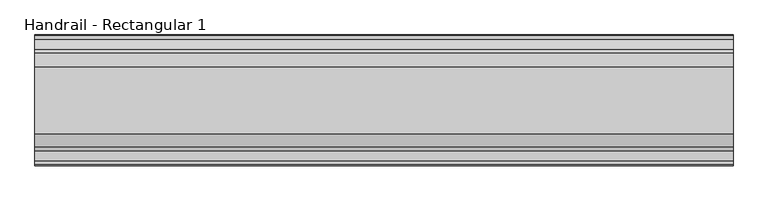
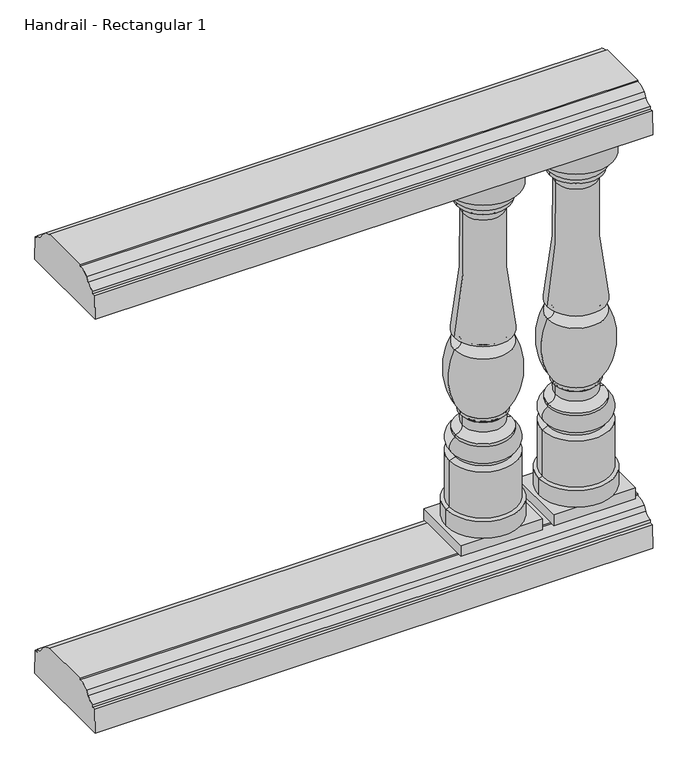
"""IFC4 building model written with IfcOpenShell, lengths in millimetres: railing geometry, Handrail - Rectangular 1."""

from ifc_helpers import new_model, si_unit, point, frame, frame_2d, origin, place, context, project, spatial, polyline, circle_curve, ellipse_curve, trimmed, segment, composite_curve, outline, extrude, source, transform, mapped, element, save
from ifc_brep_helpers import plane_surface, cylinder_surface, revolved_surface, advanced_brep


def handrail_rectangular_1_0a93f58a(model_context):
    return source(origin(), model_context, "Body", "SolidModel", [
        extrude(outline(composite_curve([segment(trimmed(circle_curve(frame_2d((-1771.1852268, 1045.36875)), 19.84375), [point((-1771.1852268, 1025.525))], [point((-1754.064785, 1035.3355607))], True, "CARTESIAN"), True, "CONTINUOUS"), segment(polyline([(-1754.064785, 1035.3355607), (-1747.604713, 1044.7951059)]), True, "CONTINUOUS"), segment(trimmed(circle_curve(frame_2d((-1723.5602268, 1018.38125)), 35.71875), [point((-1747.604713, 1044.7951059))], [point((-1723.5602268, 1054.1))], False, "CARTESIAN"), True, "CONTINUOUS"), segment(polyline([(-1723.5602268, 1054.1), (-1723.5602268, 1057.275), (-1607.6727268, 1057.275), (-1607.6727268, 1054.1)]), True, "CONTINUOUS"), segment(trimmed(circle_curve(frame_2d((-1607.6727268, 1018.38125)), 35.71875), [point((-1607.6727268, 1054.1))], [point((-1583.6282406, 1044.7951059))], False, "CARTESIAN"), True, "CONTINUOUS"), segment(polyline([(-1583.6282406, 1044.7951059), (-1577.1681686, 1035.3355607)]), True, "CONTINUOUS"), segment(trimmed(circle_curve(frame_2d((-1560.0477268, 1045.36875)), 19.84375), [point((-1577.1681686, 1035.3355607))], [point((-1560.0477268, 1025.525))], True, "CARTESIAN"), True, "CONTINUOUS"), segment(polyline([(-1560.0477268, 1025.525), (-1560.0477268, 1019.175), (-1552.9039768, 1019.175), (-1551.3164768, 965.2), (-1779.9164768, 965.2), (-1778.3289768, 1019.175), (-1771.1852268, 1019.175), (-1771.1852268, 1025.525)]), True, "CONTINUOUS")], self_intersect=False)), frame((6512.4521895, 0.0, 0.0), z_axis=(1.0, 0.0, 0.0), x_axis=(0.0, 1.0, 0.0)), (0.0, 0.0, 1.0), 1219.2),
        extrude(outline(composite_curve([segment(trimmed(circle_curve(frame_2d((-1771.1852268, 89.69375)), 19.84375), [point((-1771.1852268, 69.85))], [point((-1754.064785, 79.6605607))], True, "CARTESIAN"), True, "CONTINUOUS"), segment(polyline([(-1754.064785, 79.6605607), (-1747.604713, 89.1201059)]), True, "CONTINUOUS"), segment(trimmed(circle_curve(frame_2d((-1723.5602268, 62.70625)), 35.71875), [point((-1747.604713, 89.1201059))], [point((-1723.5602268, 98.425))], False, "CARTESIAN"), True, "CONTINUOUS"), segment(polyline([(-1723.5602268, 98.425), (-1723.5602268, 101.6), (-1607.6727268, 101.6), (-1607.6727268, 98.425)]), True, "CONTINUOUS"), segment(trimmed(circle_curve(frame_2d((-1607.6727268, 62.70625)), 35.71875), [point((-1607.6727268, 98.425))], [point((-1583.6282406, 89.1201059))], False, "CARTESIAN"), True, "CONTINUOUS"), segment(polyline([(-1583.6282406, 89.1201059), (-1577.1681686, 79.6605607)]), True, "CONTINUOUS"), segment(trimmed(circle_curve(frame_2d((-1560.0477268, 89.69375)), 19.84375), [point((-1577.1681686, 79.6605607))], [point((-1560.0477268, 69.85))], True, "CARTESIAN"), True, "CONTINUOUS"), segment(polyline([(-1560.0477268, 69.85), (-1560.0477268, 63.5), (-1552.9039768, 63.5), (-1551.3164768, 9.525), (-1779.9164768, 9.525), (-1778.3289768, 63.5), (-1771.1852268, 63.5), (-1771.1852268, 69.85)]), True, "CONTINUOUS")], self_intersect=False)), frame((6512.4521895, 0.0, 0.0), z_axis=(1.0, 0.0, 0.0), x_axis=(0.0, 1.0, 0.0)), (0.0, 0.0, 1.0), 1219.2),
        advanced_brep(
        [(7630.0521895, -1665.6164768, 939.8), (7550.6771895, -1665.6164768, 939.8), (7709.4271895, -1665.6164768, 939.8), (7711.0146895, -1665.6164768, 127.0), (7549.0896895, -1665.6164768, 127.0), (7630.0521895, -1665.6164768, 127.0), (7711.0146895, -1665.6164768, 165.2785542), (7549.0896895, -1665.6164768, 165.2785542), (7703.8709395, -1665.6164768, 168.275), (7556.2334395, -1665.6164768, 168.275), (7703.8709395, -1665.6164768, 274.7335284), (7556.2334395, -1665.6164768, 274.7335284), (7691.1709395, -1665.6164768, 280.19375), (7568.9334395, -1665.6164768, 280.19375), (7691.1709395, -1665.6164768, 286.54375), (7568.9334395, -1665.6164768, 286.54375), (7691.1709395, -1665.6164768, 324.64375), (7568.9334395, -1665.6164768, 324.64375), (7691.1709395, -1665.6164768, 330.99375), (7568.9334395, -1665.6164768, 330.99375), (7675.4640435, -1665.6164768, 347.276159), (7584.6403356, -1665.6164768, 347.276159), (7675.4640435, -1665.6164768, 368.8906259), (7584.6403356, -1665.6164768, 368.8906259), (7680.0584395, -1665.6164768, 373.85625), (7580.0459395, -1665.6164768, 373.85625), (7680.0584395, -1665.6164768, 381.4842759), (7580.0459395, -1665.6164768, 381.4842759), (7692.7584395, -1665.6164768, 527.84375), (7567.3459395, -1665.6164768, 527.84375), (7692.7584395, -1665.6164768, 556.41875), (7567.3459395, -1665.6164768, 556.41875), (7674.2243377, -1665.6164768, 836.1713606), (7585.8800414, -1665.6164768, 836.1713606), (7687.2021895, -1665.6164768, 858.04375), (7572.9021895, -1665.6164768, 858.04375), (7687.2021895, -1665.6164768, 866.775), (7572.9021895, -1665.6164768, 866.775), (7698.3146895, -1665.6164768, 892.175), (7561.7896895, -1665.6164768, 892.175), (7709.4271895, -1665.6164768, 895.35), (7550.6771895, -1665.6164768, 895.35)],
        [
            (0, 1),
            (1, 2, circle_curve(frame((7630.0521895, -1665.6164768, 939.8), z_axis=(0.0, 0.0, 1.0), x_axis=(-1.0, 0.0, 0.0)), 79.375)),
            (2, 0),
            (2, 1, circle_curve(frame((7630.0521895, -1665.6164768, 939.8), z_axis=(0.0, 0.0, 1.0), x_axis=(-1.0, 0.0, 0.0)), 79.375)),
            (3, 4, circle_curve(frame((7630.0521895, -1665.6164768, 127.0), z_axis=(0.0, 0.0, -1.0), x_axis=(-1.0, 0.0, 0.0)), 80.9625)),
            (4, 5),
            (5, 3),
            (4, 3, circle_curve(frame((7630.0521895, -1665.6164768, 127.0), z_axis=(0.0, 0.0, -1.0), x_axis=(-1.0, 0.0, 0.0)), 80.9625)),
            (6, 7, circle_curve(frame((7630.0521895, -1665.6164768, 165.2785542), z_axis=(0.0, 0.0, -1.0), x_axis=(-1.0, 0.0, 0.0)), 80.9625)),
            (7, 4),
            (3, 6),
            (7, 6, circle_curve(frame((7630.0521895, -1665.6164768, 165.2785542), z_axis=(0.0, 0.0, -1.0), x_axis=(-1.0, 0.0, 0.0)), 80.9625)),
            (8, 9, circle_curve(frame((7630.0521895, -1665.6164768, 168.275), z_axis=(0.0, 0.0, -1.0), x_axis=(-1.0, 0.0, 0.0)), 73.81875)),
            (9, 7),
            (6, 8),
            (9, 8, circle_curve(frame((7630.0521895, -1665.6164768, 168.275), z_axis=(0.0, 0.0, -1.0), x_axis=(-1.0, 0.0, 0.0)), 73.81875)),
            (10, 11, circle_curve(frame((7630.0521895, -1665.6164768, 274.7335284), z_axis=(0.0, 0.0, -1.0), x_axis=(-1.0, 0.0, 0.0)), 73.81875)),
            (11, 9),
            (8, 10),
            (11, 10, circle_curve(frame((7630.0521895, -1665.6164768, 274.7335284), z_axis=(0.0, 0.0, -1.0), x_axis=(-1.0, 0.0, 0.0)), 73.81875)),
            (12, 13, circle_curve(frame((7630.0521895, -1665.6164768, 280.19375), z_axis=(0.0, 0.0, -1.0), x_axis=(-1.0, 0.0, 0.0)), 61.11875)),
            (13, 11),
            (10, 12),
            (13, 12, circle_curve(frame((7630.0521895, -1665.6164768, 280.19375), z_axis=(0.0, 0.0, -1.0), x_axis=(-1.0, 0.0, 0.0)), 61.11875)),
            (14, 15, circle_curve(frame((7630.0521895, -1665.6164768, 286.54375), z_axis=(0.0, 0.0, -1.0), x_axis=(-1.0, 0.0, 0.0)), 61.11875)),
            (15, 13),
            (12, 14),
            (15, 14, circle_curve(frame((7630.0521895, -1665.6164768, 286.54375), z_axis=(0.0, 0.0, -1.0), x_axis=(-1.0, 0.0, 0.0)), 61.11875)),
            (16, 17, circle_curve(frame((7630.0521895, -1665.6164768, 324.64375), z_axis=(0.0, 0.0, -1.0), x_axis=(-1.0, 0.0, 0.0)), 61.11875)),
            (17, 15, circle_curve(frame((7577.1987498, -1665.6164768, 305.59375), z_axis=(0.0, -1.0, 0.0), x_axis=(1.0, 0.0, 0.0)), 20.7657856)),
            (14, 16, circle_curve(frame((7682.9056293, -1665.6164768, 305.59375), z_axis=(0.0, -1.0, 0.0), x_axis=(-1.0, 0.0, 0.0)), 20.7657856)),
            (17, 16, circle_curve(frame((7630.0521895, -1665.6164768, 324.64375), z_axis=(0.0, 0.0, -1.0), x_axis=(-1.0, 0.0, 0.0)), 61.11875)),
            (18, 19, circle_curve(frame((7630.0521895, -1665.6164768, 330.99375), z_axis=(0.0, 0.0, -1.0), x_axis=(-1.0, 0.0, 0.0)), 61.11875)),
            (19, 17),
            (16, 18),
            (19, 18, circle_curve(frame((7630.0521895, -1665.6164768, 330.99375), z_axis=(0.0, 0.0, -1.0), x_axis=(-1.0, 0.0, 0.0)), 61.11875)),
            (20, 21, circle_curve(frame((7630.0521895, -1665.6164768, 347.276159), z_axis=(0.0, 0.0, -1.0), x_axis=(-1.0, 0.0, 0.0)), 45.4118539)),
            (21, 19, circle_curve(frame((7569.4004121, -1665.6164768, 346.26035), z_axis=(0.0, 1.0, 0.0), x_axis=(1.0, 0.0, 0.0)), 15.2737402)),
            (18, 20, circle_curve(frame((7690.703967, -1665.6164768, 346.26035), z_axis=(0.0, 1.0, 0.0), x_axis=(-1.0, 0.0, 0.0)), 15.2737402)),
            (21, 20, circle_curve(frame((7630.0521895, -1665.6164768, 347.276159), z_axis=(0.0, 0.0, -1.0), x_axis=(-1.0, 0.0, 0.0)), 45.4118539)),
            (22, 23, circle_curve(frame((7630.0521895, -1665.6164768, 368.8906259), z_axis=(0.0, 0.0, -1.0), x_axis=(-1.0, 0.0, 0.0)), 45.4118539)),
            (23, 21),
            (20, 22),
            (23, 22, circle_curve(frame((7630.0521895, -1665.6164768, 368.8906259), z_axis=(0.0, 0.0, -1.0), x_axis=(-1.0, 0.0, 0.0)), 45.4118539)),
            (24, 25, circle_curve(frame((7630.0521895, -1665.6164768, 373.85625), z_axis=(0.0, 0.0, -1.0), x_axis=(-1.0, 0.0, 0.0)), 50.00625)),
            (25, 23, circle_curve(frame((7579.7940931, -1665.6164768, 369.014959), z_axis=(0.0, 1.0, 0.0), x_axis=(1.0, 0.0, 0.0)), 4.8478372)),
            (22, 24, circle_curve(frame((7680.310286, -1665.6164768, 369.014959), z_axis=(0.0, 1.0, 0.0), x_axis=(-1.0, 0.0, 0.0)), 4.8478372)),
            (25, 24, circle_curve(frame((7630.0521895, -1665.6164768, 373.85625), z_axis=(0.0, 0.0, -1.0), x_axis=(-1.0, 0.0, 0.0)), 50.00625)),
            (26, 27, circle_curve(frame((7630.0521895, -1665.6164768, 381.4842759), z_axis=(0.0, 0.0, -1.0), x_axis=(-1.0, 0.0, 0.0)), 50.00625)),
            (27, 25),
            (24, 26),
            (27, 26, circle_curve(frame((7630.0521895, -1665.6164768, 381.4842759), z_axis=(0.0, 0.0, -1.0), x_axis=(-1.0, 0.0, 0.0)), 50.00625)),
            (28, 29, circle_curve(frame((7630.0521895, -1665.6164768, 527.84375), z_axis=(0.0, 0.0, -1.0), x_axis=(-1.0, 0.0, 0.0)), 62.70625)),
            (29, 27, circle_curve(frame((7697.6829206, -1665.6164768, 465.4226923), z_axis=(0.0, -1.0, 0.0), x_axis=(1.0, 0.0, 0.0)), 144.5133802)),
            (26, 28, circle_curve(frame((7562.4214585, -1665.6164768, 465.4226923), z_axis=(0.0, -1.0, 0.0), x_axis=(-1.0, 0.0, 0.0)), 144.5133802)),
            (29, 28, circle_curve(frame((7630.0521895, -1665.6164768, 527.84375), z_axis=(0.0, 0.0, -1.0), x_axis=(-1.0, 0.0, 0.0)), 62.70625)),
            (30, 31, circle_curve(frame((7630.0521895, -1665.6164768, 556.41875), z_axis=(0.0, 0.0, -1.0), x_axis=(-1.0, 0.0, 0.0)), 62.70625)),
            (31, 29, circle_curve(frame((7568.1940628, -1665.6164768, 542.13125), z_axis=(0.0, 1.0, 0.0), x_axis=(1.0, 0.0, 0.0)), 14.3126507)),
            (28, 30, circle_curve(frame((7691.9103163, -1665.6164768, 542.13125), z_axis=(0.0, 1.0, 0.0), x_axis=(-1.0, 0.0, 0.0)), 14.3126507)),
            (31, 30, circle_curve(frame((7630.0521895, -1665.6164768, 556.41875), z_axis=(0.0, 0.0, -1.0), x_axis=(-1.0, 0.0, 0.0)), 62.70625)),
            (32, 33, circle_curve(frame((7630.0521895, -1665.6164768, 836.1713606), z_axis=(0.0, 0.0, -1.0), x_axis=(-1.0, 0.0, 0.0)), 44.1721482)),
            (33, 31, circle_curve(frame((6456.060691, -1665.6164768, 770.5336134), z_axis=(0.0, 1.0, 0.0), x_axis=(1.0, 0.0, 0.0)), 1131.7243827)),
            (30, 32, circle_curve(frame((8804.0436881, -1665.6164768, 770.5336134), z_axis=(0.0, 1.0, 0.0), x_axis=(-1.0, 0.0, 0.0)), 1131.7243827)),
            (33, 32, circle_curve(frame((7630.0521895, -1665.6164768, 836.1713606), z_axis=(0.0, 0.0, -1.0), x_axis=(-1.0, 0.0, 0.0)), 44.1721482)),
            (34, 35, circle_curve(frame((7630.0521895, -1665.6164768, 858.04375), z_axis=(0.0, 0.0, -1.0), x_axis=(-1.0, 0.0, 0.0)), 57.15)),
            (35, 33, circle_curve(frame((7564.8577367, -1665.6164768, 838.4842616), z_axis=(0.0, 1.0, 0.0), x_axis=(1.0, 0.0, 0.0)), 21.1491562)),
            (32, 34, circle_curve(frame((7695.2466424, -1665.6164768, 838.4842616), z_axis=(0.0, 1.0, 0.0), x_axis=(-1.0, 0.0, 0.0)), 21.1491562)),
            (35, 34, circle_curve(frame((7630.0521895, -1665.6164768, 858.04375), z_axis=(0.0, 0.0, -1.0), x_axis=(-1.0, 0.0, 0.0)), 57.15)),
            (36, 37, circle_curve(frame((7630.0521895, -1665.6164768, 866.775), z_axis=(0.0, 0.0, -1.0), x_axis=(-1.0, 0.0, 0.0)), 57.15)),
            (37, 35),
            (34, 36),
            (37, 36, circle_curve(frame((7630.0521895, -1665.6164768, 866.775), z_axis=(0.0, 0.0, -1.0), x_axis=(-1.0, 0.0, 0.0)), 57.15)),
            (38, 39, circle_curve(frame((7630.0521895, -1665.6164768, 892.175), z_axis=(0.0, 0.0, -1.0), x_axis=(-1.0, 0.0, 0.0)), 68.2625)),
            (39, 37, circle_curve(frame((7591.1272944, -1665.6164768, 889.8793427), z_axis=(0.0, -1.0, 0.0), x_axis=(1.0, 0.0, 0.0)), 29.4272849)),
            (36, 38, circle_curve(frame((7668.9770847, -1665.6164768, 889.8793427), z_axis=(0.0, -1.0, 0.0), x_axis=(-1.0, 0.0, 0.0)), 29.4272849)),
            (39, 38, circle_curve(frame((7630.0521895, -1665.6164768, 892.175), z_axis=(0.0, 0.0, -1.0), x_axis=(-1.0, 0.0, 0.0)), 68.2625)),
            (40, 41, circle_curve(frame((7630.0521895, -1665.6164768, 895.35), z_axis=(0.0, 0.0, -1.0), x_axis=(-1.0, 0.0, 0.0)), 79.375)),
            (41, 39),
            (38, 40),
            (41, 40, circle_curve(frame((7630.0521895, -1665.6164768, 895.35), z_axis=(0.0, 0.0, -1.0), x_axis=(-1.0, 0.0, 0.0)), 79.375)),
            (1, 41),
            (40, 2),
        ],
        [
            plane_surface(frame((7630.0521895, -1665.6164768, 939.8), z_axis=(0.0, 0.0, 1.0), x_axis=(-1.0, 0.0, 0.0))),
            plane_surface(frame((7630.0521895, -1665.6164768, 127.0), z_axis=(0.0, 0.0, -1.0), x_axis=(-1.0, 0.0, 0.0))),
            cylinder_surface(frame((7630.0521895, -1665.6164768, 1009.65), z_axis=(0.0, 0.0, 1.0), x_axis=(-1.0, 0.0, 0.0)), 80.9625),
            revolved_surface(polyline([(7549.0896895, -1665.6164768, 165.2785542), (7556.2334395, -1665.6164768, 168.275)]), (7630.0521895, -1665.6164768, 1009.65), (0.0, 0.0, 1.0)),
            cylinder_surface(frame((7630.0521895, -1665.6164768, 1009.65), z_axis=(0.0, 0.0, 1.0), x_axis=(-1.0, 0.0, 0.0)), 73.81875),
            revolved_surface(polyline([(7556.2334395, -1665.6164768, 274.7335284), (7568.9334395, -1665.6164768, 280.19375)]), (7630.0521895, -1665.6164768, 1009.65), (0.0, 0.0, 1.0)),
            cylinder_surface(frame((7630.0521895, -1665.6164768, 1009.65), z_axis=(0.0, 0.0, 1.0), x_axis=(-1.0, 0.0, 0.0)), 61.11875),
            revolved_surface(trimmed(ellipse_curve(frame((7577.1987498, -1665.6164768, 305.59375), z_axis=(0.0, 1.0, 0.0), x_axis=(1.0, 0.0, 0.0)), 20.7657856, 20.7657856), [point((7568.9334395, -1665.6164768, 286.54375))], [point((7568.9334395, -1665.6164768, 324.64375))], True, "CARTESIAN"), (7630.0521895, -1665.6164768, 1009.65), (0.0, 0.0, 1.0)),
            revolved_surface(trimmed(ellipse_curve(frame((7569.4004121, -1665.6164768, 346.26035), z_axis=(0.0, -1.0, 0.0), x_axis=(1.0, 0.0, 0.0)), 15.2737402, 15.2737402), [point((7568.9334395, -1665.6164768, 330.99375))], [point((7584.6403356, -1665.6164768, 347.276159))], True, "CARTESIAN"), (7630.0521895, -1665.6164768, 1009.65), (0.0, 0.0, 1.0)),
            cylinder_surface(frame((7630.0521895, -1665.6164768, 1009.65), z_axis=(0.0, 0.0, 1.0), x_axis=(-1.0, 0.0, 0.0)), 45.4118539),
            revolved_surface(trimmed(ellipse_curve(frame((7579.7940931, -1665.6164768, 369.014959), z_axis=(0.0, -1.0, 0.0), x_axis=(1.0, 0.0, 0.0)), 4.8478372, 4.8478372), [point((7584.6403356, -1665.6164768, 368.8906259))], [point((7580.0459395, -1665.6164768, 373.85625))], True, "CARTESIAN"), (7630.0521895, -1665.6164768, 1009.65), (0.0, 0.0, 1.0)),
            cylinder_surface(frame((7630.0521895, -1665.6164768, 1009.65), z_axis=(0.0, 0.0, 1.0), x_axis=(-1.0, 0.0, 0.0)), 50.00625),
            revolved_surface(trimmed(ellipse_curve(frame((7697.6829206, -1665.6164768, 465.4226923), z_axis=(0.0, 1.0, 0.0), x_axis=(1.0, 0.0, 0.0)), 144.5133802, 144.5133802), [point((7580.0459395, -1665.6164768, 381.4842759))], [point((7567.3459395, -1665.6164768, 527.84375))], True, "CARTESIAN"), (7630.0521895, -1665.6164768, 1009.65), (0.0, 0.0, 1.0)),
            revolved_surface(trimmed(ellipse_curve(frame((7568.1940628, -1665.6164768, 542.13125), z_axis=(0.0, -1.0, 0.0), x_axis=(1.0, 0.0, 0.0)), 14.3126507, 14.3126507), [point((7567.3459395, -1665.6164768, 527.84375))], [point((7567.3459395, -1665.6164768, 556.41875))], True, "CARTESIAN"), (7630.0521895, -1665.6164768, 1009.65), (0.0, 0.0, 1.0)),
            revolved_surface(trimmed(ellipse_curve(frame((6456.060691, -1665.6164768, 770.5336134), z_axis=(0.0, -1.0, 0.0), x_axis=(1.0, 0.0, 0.0)), 1131.7243827, 1131.7243827), [point((7567.3459395, -1665.6164768, 556.41875))], [point((7585.8800414, -1665.6164768, 836.1713606))], True, "CARTESIAN"), (7630.0521895, -1665.6164768, 1009.65), (0.0, 0.0, 1.0)),
            revolved_surface(trimmed(ellipse_curve(frame((7564.8577367, -1665.6164768, 838.4842616), z_axis=(0.0, -1.0, 0.0), x_axis=(1.0, 0.0, 0.0)), 21.1491562, 21.1491562), [point((7585.8800414, -1665.6164768, 836.1713606))], [point((7572.9021895, -1665.6164768, 858.04375))], True, "CARTESIAN"), (7630.0521895, -1665.6164768, 1009.65), (0.0, 0.0, 1.0)),
            cylinder_surface(frame((7630.0521895, -1665.6164768, 1009.65), z_axis=(0.0, 0.0, 1.0), x_axis=(-1.0, 0.0, 0.0)), 57.15),
            revolved_surface(trimmed(ellipse_curve(frame((7591.1272944, -1665.6164768, 889.8793427), z_axis=(0.0, 1.0, 0.0), x_axis=(1.0, 0.0, 0.0)), 29.4272849, 29.4272849), [point((7572.9021895, -1665.6164768, 866.775))], [point((7561.7896895, -1665.6164768, 892.175))], True, "CARTESIAN"), (7630.0521895, -1665.6164768, 1009.65), (0.0, 0.0, 1.0)),
            revolved_surface(polyline([(7561.7896895, -1665.6164768, 892.175), (7550.6771895, -1665.6164768, 895.35)]), (7630.0521895, -1665.6164768, 1009.65), (0.0, 0.0, 1.0)),
            cylinder_surface(frame((7630.0521895, -1665.6164768, 1009.65), z_axis=(0.0, 0.0, 1.0), x_axis=(-1.0, 0.0, 0.0)), 79.375),
        ],
        [
            (0, [[1, 2, 3]]),
            (0, [[-3, 4, -1]]),
            (1, [[5, 6, 7]]),
            (1, [[8, -7, -6]]),
            (2, [[9, 10, -5, 11]]),
            (2, [[12, -11, -8, -10]]),
            (3, [[13, 14, -9, 15]]),
            (3, [[16, -15, -12, -14]]),
            (4, [[17, 18, -13, 19]]),
            (4, [[20, -19, -16, -18]]),
            (5, [[21, 22, -17, 23]]),
            (5, [[24, -23, -20, -22]]),
            (6, [[25, 26, -21, 27]]),
            (6, [[28, -27, -24, -26]]),
            (7, [[29, 30, -25, 31]]),
            (7, [[32, -31, -28, -30]]),
            (6, [[33, 34, -29, 35]]),
            (6, [[36, -35, -32, -34]]),
            (8, [[37, 38, -33, 39]]),
            (8, [[40, -39, -36, -38]]),
            (9, [[41, 42, -37, 43]]),
            (9, [[44, -43, -40, -42]]),
            (10, [[45, 46, -41, 47]]),
            (10, [[48, -47, -44, -46]]),
            (11, [[49, 50, -45, 51]]),
            (11, [[52, -51, -48, -50]]),
            (12, [[53, 54, -49, 55]]),
            (12, [[56, -55, -52, -54]]),
            (13, [[57, 58, -53, 59]]),
            (13, [[60, -59, -56, -58]]),
            (14, [[61, 62, -57, 63]]),
            (14, [[64, -63, -60, -62]]),
            (15, [[65, 66, -61, 67]]),
            (15, [[68, -67, -64, -66]]),
            (16, [[69, 70, -65, 71]]),
            (16, [[72, -71, -68, -70]]),
            (17, [[73, 74, -69, 75]]),
            (17, [[76, -75, -72, -74]]),
            (18, [[77, 78, -73, 79]]),
            (18, [[80, -79, -76, -78]]),
            (19, [[-2, 81, -77, 82]]),
            (19, [[-4, -82, -80, -81]]),
        ],
    ),
        extrude(outline(polyline([(7541.1521895, -1735.4664768), (7541.1521895, -1595.7664768), (7718.9521895, -1595.7664768), (7718.9521895, -1735.4664768), (7541.1521895, -1735.4664768)])), frame((0.0, 0.0, 101.6), z_axis=(0.0, 0.0, 1.0), x_axis=(1.0, 0.0, 0.0)), (0.0, 0.0, 1.0), 25.4),
        extrude(outline(polyline([(7541.1521895, -1595.7664768), (7718.9521895, -1595.7664768), (7718.9521895, -1735.4664768), (7541.1521895, -1735.4664768), (7541.1521895, -1595.7664768)])), frame((0.0, 0.0, 939.8), z_axis=(0.0, 0.0, 1.0), x_axis=(1.0, 0.0, 0.0)), (0.0, 0.0, 1.0), 25.4),
        advanced_brep(
        [(7426.8521895, -1665.6164768, 939.8), (7347.4771895, -1665.6164768, 939.8), (7506.2271895, -1665.6164768, 939.8), (7507.8146895, -1665.6164768, 127.0), (7345.8896895, -1665.6164768, 127.0), (7426.8521895, -1665.6164768, 127.0), (7507.8146895, -1665.6164768, 165.2785542), (7345.8896895, -1665.6164768, 165.2785542), (7500.6709395, -1665.6164768, 168.275), (7353.0334395, -1665.6164768, 168.275), (7500.6709395, -1665.6164768, 274.7335284), (7353.0334395, -1665.6164768, 274.7335284), (7487.9709395, -1665.6164768, 280.19375), (7365.7334395, -1665.6164768, 280.19375), (7487.9709395, -1665.6164768, 286.54375), (7365.7334395, -1665.6164768, 286.54375), (7487.9709395, -1665.6164768, 324.64375), (7365.7334395, -1665.6164768, 324.64375), (7487.9709395, -1665.6164768, 330.99375), (7365.7334395, -1665.6164768, 330.99375), (7472.2640435, -1665.6164768, 347.276159), (7381.4403356, -1665.6164768, 347.276159), (7472.2640435, -1665.6164768, 368.8906259), (7381.4403356, -1665.6164768, 368.8906259), (7476.8584395, -1665.6164768, 373.85625), (7376.8459395, -1665.6164768, 373.85625), (7476.8584395, -1665.6164768, 381.4842759), (7376.8459395, -1665.6164768, 381.4842759), (7489.5584395, -1665.6164768, 527.84375), (7364.1459395, -1665.6164768, 527.84375), (7489.5584395, -1665.6164768, 556.41875), (7364.1459395, -1665.6164768, 556.41875), (7471.0243377, -1665.6164768, 836.1713606), (7382.6800414, -1665.6164768, 836.1713606), (7484.0021895, -1665.6164768, 858.04375), (7369.7021895, -1665.6164768, 858.04375), (7484.0021895, -1665.6164768, 866.775), (7369.7021895, -1665.6164768, 866.775), (7495.1146895, -1665.6164768, 892.175), (7358.5896895, -1665.6164768, 892.175), (7506.2271895, -1665.6164768, 895.35), (7347.4771895, -1665.6164768, 895.35)],
        [
            (0, 1),
            (1, 2, circle_curve(frame((7426.8521895, -1665.6164768, 939.8), z_axis=(0.0, 0.0, 1.0), x_axis=(-1.0, 0.0, 0.0)), 79.375)),
            (2, 0),
            (2, 1, circle_curve(frame((7426.8521895, -1665.6164768, 939.8), z_axis=(0.0, 0.0, 1.0), x_axis=(-1.0, 0.0, 0.0)), 79.375)),
            (3, 4, circle_curve(frame((7426.8521895, -1665.6164768, 127.0), z_axis=(0.0, 0.0, -1.0), x_axis=(-1.0, 0.0, 0.0)), 80.9625)),
            (4, 5),
            (5, 3),
            (4, 3, circle_curve(frame((7426.8521895, -1665.6164768, 127.0), z_axis=(0.0, 0.0, -1.0), x_axis=(-1.0, 0.0, 0.0)), 80.9625)),
            (6, 7, circle_curve(frame((7426.8521895, -1665.6164768, 165.2785542), z_axis=(0.0, 0.0, -1.0), x_axis=(-1.0, 0.0, 0.0)), 80.9625)),
            (7, 4),
            (3, 6),
            (7, 6, circle_curve(frame((7426.8521895, -1665.6164768, 165.2785542), z_axis=(0.0, 0.0, -1.0), x_axis=(-1.0, 0.0, 0.0)), 80.9625)),
            (8, 9, circle_curve(frame((7426.8521895, -1665.6164768, 168.275), z_axis=(0.0, 0.0, -1.0), x_axis=(-1.0, 0.0, 0.0)), 73.81875)),
            (9, 7),
            (6, 8),
            (9, 8, circle_curve(frame((7426.8521895, -1665.6164768, 168.275), z_axis=(0.0, 0.0, -1.0), x_axis=(-1.0, 0.0, 0.0)), 73.81875)),
            (10, 11, circle_curve(frame((7426.8521895, -1665.6164768, 274.7335284), z_axis=(0.0, 0.0, -1.0), x_axis=(-1.0, 0.0, 0.0)), 73.81875)),
            (11, 9),
            (8, 10),
            (11, 10, circle_curve(frame((7426.8521895, -1665.6164768, 274.7335284), z_axis=(0.0, 0.0, -1.0), x_axis=(-1.0, 0.0, 0.0)), 73.81875)),
            (12, 13, circle_curve(frame((7426.8521895, -1665.6164768, 280.19375), z_axis=(0.0, 0.0, -1.0), x_axis=(-1.0, 0.0, 0.0)), 61.11875)),
            (13, 11),
            (10, 12),
            (13, 12, circle_curve(frame((7426.8521895, -1665.6164768, 280.19375), z_axis=(0.0, 0.0, -1.0), x_axis=(-1.0, 0.0, 0.0)), 61.11875)),
            (14, 15, circle_curve(frame((7426.8521895, -1665.6164768, 286.54375), z_axis=(0.0, 0.0, -1.0), x_axis=(-1.0, 0.0, 0.0)), 61.11875)),
            (15, 13),
            (12, 14),
            (15, 14, circle_curve(frame((7426.8521895, -1665.6164768, 286.54375), z_axis=(0.0, 0.0, -1.0), x_axis=(-1.0, 0.0, 0.0)), 61.11875)),
            (16, 17, circle_curve(frame((7426.8521895, -1665.6164768, 324.64375), z_axis=(0.0, 0.0, -1.0), x_axis=(-1.0, 0.0, 0.0)), 61.11875)),
            (17, 15, circle_curve(frame((7373.9987498, -1665.6164768, 305.59375), z_axis=(0.0, -1.0, 0.0), x_axis=(1.0, 0.0, 0.0)), 20.7657856)),
            (14, 16, circle_curve(frame((7479.7056293, -1665.6164768, 305.59375), z_axis=(0.0, -1.0, 0.0), x_axis=(-1.0, 0.0, 0.0)), 20.7657856)),
            (17, 16, circle_curve(frame((7426.8521895, -1665.6164768, 324.64375), z_axis=(0.0, 0.0, -1.0), x_axis=(-1.0, 0.0, 0.0)), 61.11875)),
            (18, 19, circle_curve(frame((7426.8521895, -1665.6164768, 330.99375), z_axis=(0.0, 0.0, -1.0), x_axis=(-1.0, 0.0, 0.0)), 61.11875)),
            (19, 17),
            (16, 18),
            (19, 18, circle_curve(frame((7426.8521895, -1665.6164768, 330.99375), z_axis=(0.0, 0.0, -1.0), x_axis=(-1.0, 0.0, 0.0)), 61.11875)),
            (20, 21, circle_curve(frame((7426.8521895, -1665.6164768, 347.276159), z_axis=(0.0, 0.0, -1.0), x_axis=(-1.0, 0.0, 0.0)), 45.4118539)),
            (21, 19, circle_curve(frame((7366.2004121, -1665.6164768, 346.26035), z_axis=(0.0, 1.0, 0.0), x_axis=(1.0, 0.0, 0.0)), 15.2737402)),
            (18, 20, circle_curve(frame((7487.503967, -1665.6164768, 346.26035), z_axis=(0.0, 1.0, 0.0), x_axis=(-1.0, 0.0, 0.0)), 15.2737402)),
            (21, 20, circle_curve(frame((7426.8521895, -1665.6164768, 347.276159), z_axis=(0.0, 0.0, -1.0), x_axis=(-1.0, 0.0, 0.0)), 45.4118539)),
            (22, 23, circle_curve(frame((7426.8521895, -1665.6164768, 368.8906259), z_axis=(0.0, 0.0, -1.0), x_axis=(-1.0, 0.0, 0.0)), 45.4118539)),
            (23, 21),
            (20, 22),
            (23, 22, circle_curve(frame((7426.8521895, -1665.6164768, 368.8906259), z_axis=(0.0, 0.0, -1.0), x_axis=(-1.0, 0.0, 0.0)), 45.4118539)),
            (24, 25, circle_curve(frame((7426.8521895, -1665.6164768, 373.85625), z_axis=(0.0, 0.0, -1.0), x_axis=(-1.0, 0.0, 0.0)), 50.00625)),
            (25, 23, circle_curve(frame((7376.5940931, -1665.6164768, 369.014959), z_axis=(0.0, 1.0, 0.0), x_axis=(1.0, 0.0, 0.0)), 4.8478372)),
            (22, 24, circle_curve(frame((7477.110286, -1665.6164768, 369.014959), z_axis=(0.0, 1.0, 0.0), x_axis=(-1.0, 0.0, 0.0)), 4.8478372)),
            (25, 24, circle_curve(frame((7426.8521895, -1665.6164768, 373.85625), z_axis=(0.0, 0.0, -1.0), x_axis=(-1.0, 0.0, 0.0)), 50.00625)),
            (26, 27, circle_curve(frame((7426.8521895, -1665.6164768, 381.4842759), z_axis=(0.0, 0.0, -1.0), x_axis=(-1.0, 0.0, 0.0)), 50.00625)),
            (27, 25),
            (24, 26),
            (27, 26, circle_curve(frame((7426.8521895, -1665.6164768, 381.4842759), z_axis=(0.0, 0.0, -1.0), x_axis=(-1.0, 0.0, 0.0)), 50.00625)),
            (28, 29, circle_curve(frame((7426.8521895, -1665.6164768, 527.84375), z_axis=(0.0, 0.0, -1.0), x_axis=(-1.0, 0.0, 0.0)), 62.70625)),
            (29, 27, circle_curve(frame((7494.4829206, -1665.6164768, 465.4226923), z_axis=(0.0, -1.0, 0.0), x_axis=(1.0, 0.0, 0.0)), 144.5133802)),
            (26, 28, circle_curve(frame((7359.2214585, -1665.6164768, 465.4226923), z_axis=(0.0, -1.0, 0.0), x_axis=(-1.0, 0.0, 0.0)), 144.5133802)),
            (29, 28, circle_curve(frame((7426.8521895, -1665.6164768, 527.84375), z_axis=(0.0, 0.0, -1.0), x_axis=(-1.0, 0.0, 0.0)), 62.70625)),
            (30, 31, circle_curve(frame((7426.8521895, -1665.6164768, 556.41875), z_axis=(0.0, 0.0, -1.0), x_axis=(-1.0, 0.0, 0.0)), 62.70625)),
            (31, 29, circle_curve(frame((7364.9940628, -1665.6164768, 542.13125), z_axis=(0.0, 1.0, 0.0), x_axis=(1.0, 0.0, 0.0)), 14.3126507)),
            (28, 30, circle_curve(frame((7488.7103163, -1665.6164768, 542.13125), z_axis=(0.0, 1.0, 0.0), x_axis=(-1.0, 0.0, 0.0)), 14.3126507)),
            (31, 30, circle_curve(frame((7426.8521895, -1665.6164768, 556.41875), z_axis=(0.0, 0.0, -1.0), x_axis=(-1.0, 0.0, 0.0)), 62.70625)),
            (32, 33, circle_curve(frame((7426.8521895, -1665.6164768, 836.1713606), z_axis=(0.0, 0.0, -1.0), x_axis=(-1.0, 0.0, 0.0)), 44.1721482)),
            (33, 31, circle_curve(frame((6252.860691, -1665.6164768, 770.5336134), z_axis=(0.0, 1.0, 0.0), x_axis=(1.0, 0.0, 0.0)), 1131.7243827)),
            (30, 32, circle_curve(frame((8600.8436881, -1665.6164768, 770.5336134), z_axis=(0.0, 1.0, 0.0), x_axis=(-1.0, 0.0, 0.0)), 1131.7243827)),
            (33, 32, circle_curve(frame((7426.8521895, -1665.6164768, 836.1713606), z_axis=(0.0, 0.0, -1.0), x_axis=(-1.0, 0.0, 0.0)), 44.1721482)),
            (34, 35, circle_curve(frame((7426.8521895, -1665.6164768, 858.04375), z_axis=(0.0, 0.0, -1.0), x_axis=(-1.0, 0.0, 0.0)), 57.15)),
            (35, 33, circle_curve(frame((7361.6577367, -1665.6164768, 838.4842616), z_axis=(0.0, 1.0, 0.0), x_axis=(1.0, 0.0, 0.0)), 21.1491562)),
            (32, 34, circle_curve(frame((7492.0466424, -1665.6164768, 838.4842616), z_axis=(0.0, 1.0, 0.0), x_axis=(-1.0, 0.0, 0.0)), 21.1491562)),
            (35, 34, circle_curve(frame((7426.8521895, -1665.6164768, 858.04375), z_axis=(0.0, 0.0, -1.0), x_axis=(-1.0, 0.0, 0.0)), 57.15)),
            (36, 37, circle_curve(frame((7426.8521895, -1665.6164768, 866.775), z_axis=(0.0, 0.0, -1.0), x_axis=(-1.0, 0.0, 0.0)), 57.15)),
            (37, 35),
            (34, 36),
            (37, 36, circle_curve(frame((7426.8521895, -1665.6164768, 866.775), z_axis=(0.0, 0.0, -1.0), x_axis=(-1.0, 0.0, 0.0)), 57.15)),
            (38, 39, circle_curve(frame((7426.8521895, -1665.6164768, 892.175), z_axis=(0.0, 0.0, -1.0), x_axis=(-1.0, 0.0, 0.0)), 68.2625)),
            (39, 37, circle_curve(frame((7387.9272944, -1665.6164768, 889.8793427), z_axis=(0.0, -1.0, 0.0), x_axis=(1.0, 0.0, 0.0)), 29.4272849)),
            (36, 38, circle_curve(frame((7465.7770847, -1665.6164768, 889.8793427), z_axis=(0.0, -1.0, 0.0), x_axis=(-1.0, 0.0, 0.0)), 29.4272849)),
            (39, 38, circle_curve(frame((7426.8521895, -1665.6164768, 892.175), z_axis=(0.0, 0.0, -1.0), x_axis=(-1.0, 0.0, 0.0)), 68.2625)),
            (40, 41, circle_curve(frame((7426.8521895, -1665.6164768, 895.35), z_axis=(0.0, 0.0, -1.0), x_axis=(-1.0, 0.0, 0.0)), 79.375)),
            (41, 39),
            (38, 40),
            (41, 40, circle_curve(frame((7426.8521895, -1665.6164768, 895.35), z_axis=(0.0, 0.0, -1.0), x_axis=(-1.0, 0.0, 0.0)), 79.375)),
            (1, 41),
            (40, 2),
        ],
        [
            plane_surface(frame((7426.8521895, -1665.6164768, 939.8), z_axis=(0.0, 0.0, 1.0), x_axis=(-1.0, 0.0, 0.0))),
            plane_surface(frame((7426.8521895, -1665.6164768, 127.0), z_axis=(0.0, 0.0, -1.0), x_axis=(-1.0, 0.0, 0.0))),
            cylinder_surface(frame((7426.8521895, -1665.6164768, 1009.65), z_axis=(0.0, 0.0, 1.0), x_axis=(-1.0, 0.0, 0.0)), 80.9625),
            revolved_surface(polyline([(7345.8896895, -1665.6164768, 165.2785542), (7353.0334395, -1665.6164768, 168.275)]), (7426.8521895, -1665.6164768, 1009.65), (0.0, 0.0, 1.0)),
            cylinder_surface(frame((7426.8521895, -1665.6164768, 1009.65), z_axis=(0.0, 0.0, 1.0), x_axis=(-1.0, 0.0, 0.0)), 73.81875),
            revolved_surface(polyline([(7353.0334395, -1665.6164768, 274.7335284), (7365.7334395, -1665.6164768, 280.19375)]), (7426.8521895, -1665.6164768, 1009.65), (0.0, 0.0, 1.0)),
            cylinder_surface(frame((7426.8521895, -1665.6164768, 1009.65), z_axis=(0.0, 0.0, 1.0), x_axis=(-1.0, 0.0, 0.0)), 61.11875),
            revolved_surface(trimmed(ellipse_curve(frame((7373.9987498, -1665.6164768, 305.59375), z_axis=(0.0, 1.0, 0.0), x_axis=(1.0, 0.0, 0.0)), 20.7657856, 20.7657856), [point((7365.7334395, -1665.6164768, 286.54375))], [point((7365.7334395, -1665.6164768, 324.64375))], True, "CARTESIAN"), (7426.8521895, -1665.6164768, 1009.65), (0.0, 0.0, 1.0)),
            revolved_surface(trimmed(ellipse_curve(frame((7366.2004121, -1665.6164768, 346.26035), z_axis=(0.0, -1.0, 0.0), x_axis=(1.0, 0.0, 0.0)), 15.2737402, 15.2737402), [point((7365.7334395, -1665.6164768, 330.99375))], [point((7381.4403356, -1665.6164768, 347.276159))], True, "CARTESIAN"), (7426.8521895, -1665.6164768, 1009.65), (0.0, 0.0, 1.0)),
            cylinder_surface(frame((7426.8521895, -1665.6164768, 1009.65), z_axis=(0.0, 0.0, 1.0), x_axis=(-1.0, 0.0, 0.0)), 45.4118539),
            revolved_surface(trimmed(ellipse_curve(frame((7376.5940931, -1665.6164768, 369.014959), z_axis=(0.0, -1.0, 0.0), x_axis=(1.0, 0.0, 0.0)), 4.8478372, 4.8478372), [point((7381.4403356, -1665.6164768, 368.8906259))], [point((7376.8459395, -1665.6164768, 373.85625))], True, "CARTESIAN"), (7426.8521895, -1665.6164768, 1009.65), (0.0, 0.0, 1.0)),
            cylinder_surface(frame((7426.8521895, -1665.6164768, 1009.65), z_axis=(0.0, 0.0, 1.0), x_axis=(-1.0, 0.0, 0.0)), 50.00625),
            revolved_surface(trimmed(ellipse_curve(frame((7494.4829206, -1665.6164768, 465.4226923), z_axis=(0.0, 1.0, 0.0), x_axis=(1.0, 0.0, 0.0)), 144.5133802, 144.5133802), [point((7376.8459395, -1665.6164768, 381.4842759))], [point((7364.1459395, -1665.6164768, 527.84375))], True, "CARTESIAN"), (7426.8521895, -1665.6164768, 1009.65), (0.0, 0.0, 1.0)),
            revolved_surface(trimmed(ellipse_curve(frame((7364.9940628, -1665.6164768, 542.13125), z_axis=(0.0, -1.0, 0.0), x_axis=(1.0, 0.0, 0.0)), 14.3126507, 14.3126507), [point((7364.1459395, -1665.6164768, 527.84375))], [point((7364.1459395, -1665.6164768, 556.41875))], True, "CARTESIAN"), (7426.8521895, -1665.6164768, 1009.65), (0.0, 0.0, 1.0)),
            revolved_surface(trimmed(ellipse_curve(frame((6252.860691, -1665.6164768, 770.5336134), z_axis=(0.0, -1.0, 0.0), x_axis=(1.0, 0.0, 0.0)), 1131.7243827, 1131.7243827), [point((7364.1459395, -1665.6164768, 556.41875))], [point((7382.6800414, -1665.6164768, 836.1713606))], True, "CARTESIAN"), (7426.8521895, -1665.6164768, 1009.65), (0.0, 0.0, 1.0)),
            revolved_surface(trimmed(ellipse_curve(frame((7361.6577367, -1665.6164768, 838.4842616), z_axis=(0.0, -1.0, 0.0), x_axis=(1.0, 0.0, 0.0)), 21.1491562, 21.1491562), [point((7382.6800414, -1665.6164768, 836.1713606))], [point((7369.7021895, -1665.6164768, 858.04375))], True, "CARTESIAN"), (7426.8521895, -1665.6164768, 1009.65), (0.0, 0.0, 1.0)),
            cylinder_surface(frame((7426.8521895, -1665.6164768, 1009.65), z_axis=(0.0, 0.0, 1.0), x_axis=(-1.0, 0.0, 0.0)), 57.15),
            revolved_surface(trimmed(ellipse_curve(frame((7387.9272944, -1665.6164768, 889.8793427), z_axis=(0.0, 1.0, 0.0), x_axis=(1.0, 0.0, 0.0)), 29.4272849, 29.4272849), [point((7369.7021895, -1665.6164768, 866.775))], [point((7358.5896895, -1665.6164768, 892.175))], True, "CARTESIAN"), (7426.8521895, -1665.6164768, 1009.65), (0.0, 0.0, 1.0)),
            revolved_surface(polyline([(7358.5896895, -1665.6164768, 892.175), (7347.4771895, -1665.6164768, 895.35)]), (7426.8521895, -1665.6164768, 1009.65), (0.0, 0.0, 1.0)),
            cylinder_surface(frame((7426.8521895, -1665.6164768, 1009.65), z_axis=(0.0, 0.0, 1.0), x_axis=(-1.0, 0.0, 0.0)), 79.375),
        ],
        [
            (0, [[1, 2, 3]]),
            (0, [[-3, 4, -1]]),
            (1, [[5, 6, 7]]),
            (1, [[8, -7, -6]]),
            (2, [[9, 10, -5, 11]]),
            (2, [[12, -11, -8, -10]]),
            (3, [[13, 14, -9, 15]]),
            (3, [[16, -15, -12, -14]]),
            (4, [[17, 18, -13, 19]]),
            (4, [[20, -19, -16, -18]]),
            (5, [[21, 22, -17, 23]]),
            (5, [[24, -23, -20, -22]]),
            (6, [[25, 26, -21, 27]]),
            (6, [[28, -27, -24, -26]]),
            (7, [[29, 30, -25, 31]]),
            (7, [[32, -31, -28, -30]]),
            (6, [[33, 34, -29, 35]]),
            (6, [[36, -35, -32, -34]]),
            (8, [[37, 38, -33, 39]]),
            (8, [[40, -39, -36, -38]]),
            (9, [[41, 42, -37, 43]]),
            (9, [[44, -43, -40, -42]]),
            (10, [[45, 46, -41, 47]]),
            (10, [[48, -47, -44, -46]]),
            (11, [[49, 50, -45, 51]]),
            (11, [[52, -51, -48, -50]]),
            (12, [[53, 54, -49, 55]]),
            (12, [[56, -55, -52, -54]]),
            (13, [[57, 58, -53, 59]]),
            (13, [[60, -59, -56, -58]]),
            (14, [[61, 62, -57, 63]]),
            (14, [[64, -63, -60, -62]]),
            (15, [[65, 66, -61, 67]]),
            (15, [[68, -67, -64, -66]]),
            (16, [[69, 70, -65, 71]]),
            (16, [[72, -71, -68, -70]]),
            (17, [[73, 74, -69, 75]]),
            (17, [[76, -75, -72, -74]]),
            (18, [[77, 78, -73, 79]]),
            (18, [[80, -79, -76, -78]]),
            (19, [[-2, 81, -77, 82]]),
            (19, [[-4, -82, -80, -81]]),
        ],
    ),
        extrude(outline(polyline([(7337.9521895, -1735.4664768), (7337.9521895, -1595.7664768), (7515.7521895, -1595.7664768), (7515.7521895, -1735.4664768), (7337.9521895, -1735.4664768)])), frame((0.0, 0.0, 101.6), z_axis=(0.0, 0.0, 1.0), x_axis=(1.0, 0.0, 0.0)), (0.0, 0.0, 1.0), 25.4),
        extrude(outline(polyline([(7337.9521895, -1595.7664768), (7515.7521895, -1595.7664768), (7515.7521895, -1735.4664768), (7337.9521895, -1735.4664768), (7337.9521895, -1595.7664768)])), frame((0.0, 0.0, 939.8), z_axis=(0.0, 0.0, 1.0), x_axis=(1.0, 0.0, 0.0)), (0.0, 0.0, 1.0), 25.4),
    ])


if __name__ == "__main__":
    model = new_model("IFC4")
    model_context = context("Model", 3, world=origin())
    ifc_project = project(units=[si_unit("LENGTHUNIT", "METRE", prefix="MILLI")], contexts=[model_context])
    site = spatial("IfcSite", under=ifc_project)
    building = spatial("IfcBuilding", under=site)
    placement = place(None, origin())
    handrail_rectangular_1_shape = handrail_rectangular_1_0a93f58a(model_context)
    element("IfcRailing", 1, ObjectType="Handrail - Rectangular 1", at=placement, inside=building, context=model_context, shape_type="MappedRepresentation", body=[
        mapped(handrail_rectangular_1_shape, transform((0.0, 0.0, 0.0), x_axis=(1.0, 0.0, 0.0), y_axis=(0.0, 1.0, 0.0), z_axis=(0.0, 0.0, 1.0))),
    ])
    save(model, "model.ifc")

# Revit data of these elements
# Project information
#   Project Issue Date = "Issue Date"
#   Project Status = "Project Status"
#   Client Name = "Owner"
#   Project Address = "Enter address here"
#   Project Name = "Project Name"
#   Project Number = "Project Number"
